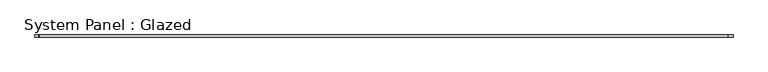
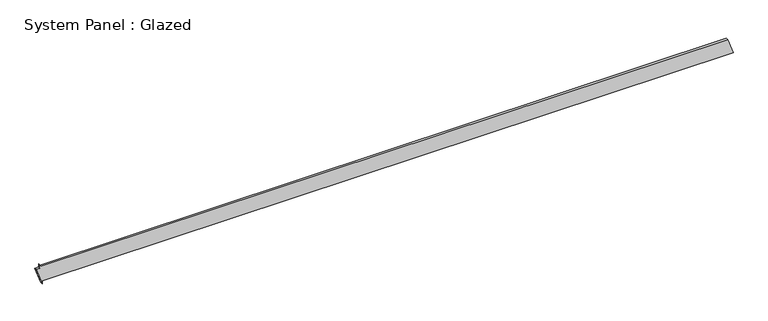
"""IFC4 building model written with IfcOpenShell, lengths in millimetres: plate geometry, System Panel : Glazed."""

from ifc_helpers import new_model, si_unit, frame, origin, place, context, project, spatial, polyline, outline, extrude, source, transform, mapped, element, save


def system_panel_glazed_8c59b1fc(model_context):
    return source(origin(), model_context, "Body", "SweptSolid", [
        extrude(outline(polyline([(0.0, -3958.9006636), (35.3553391, -3958.9006636), (35.3553391, 4028.2357193), (216.08316, 3965.7843314), (216.0411342, -3974.3837815), (235.4832574, -3985.250862), (200.1279184, -3985.250658), (200.1276704, -4028.2357193), (0.0, -3958.9006636)])), frame((0.0, -49.5, 0.0), z_axis=(0.0, 1.0, 0.0), x_axis=(0.0, 0.0, 1.0)), (0.0, 0.0, 1.0), 25.0),
    ])


if __name__ == "__main__":
    model = new_model("IFC4")
    model_context = context("Model", 3, world=origin())
    ifc_project = project(units=[si_unit("LENGTHUNIT", "METRE", prefix="MILLI")], contexts=[model_context])
    site = spatial("IfcSite", under=ifc_project)
    building = spatial("IfcBuilding", under=site)
    placement = place(None, origin())
    system_panel_glazed_shape = system_panel_glazed_8c59b1fc(model_context)
    element("IfcPlate", 1, ObjectType="System Panel : Glazed", at=placement, inside=building, context=model_context, shape_type="MappedRepresentation", body=[
        mapped(system_panel_glazed_shape, transform((0.0, 0.0, 0.0), x_axis=(1.0, 0.0, 0.0), y_axis=(0.0, 1.0, 0.0), z_axis=(0.0, 0.0, 1.0))),
    ])
    save(model, "model.ifc")

# Revit data of these elements
# Element 1 (IfcPlate, "System Panel : Glazed")
#   Materials on its faces: "Glass"
# Materials
#   "Glass": class "Glass", colour RGB 218 227 224, transparency 0.85, Description = "Soda Lime Glass", Cost = 0
